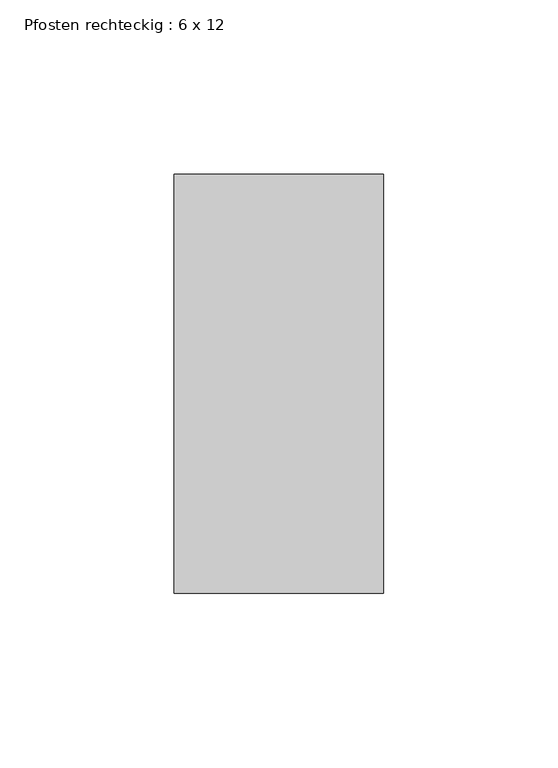
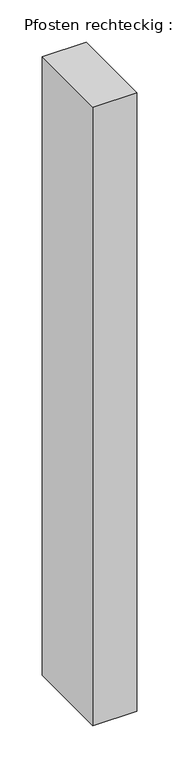
"""IFC4 building model written with IfcOpenShell, lengths in millimetres: member geometry, Pfosten rechteckig : 6 x 12."""

from ifc_helpers import new_model, si_unit, frame, origin, place, context, project, spatial, polyline, outline, extrude, source, transform, mapped, element, save


def pfosten_rechteckig_6_x_12_970216da(model_context):
    return source(origin(), model_context, "Body", "SweptSolid", [
        extrude(outline(polyline([(30.0, 60.0), (30.0, -60.0), (-30.0, -60.0), (-30.0, 60.0), (30.0, 60.0)])), frame((0.0, 0.0, -895.0226945), z_axis=(0.0, 0.0, 1.0), x_axis=(1.0, 0.0, 0.0)), (0.0, 0.0, 1.0), 895.0226945),
    ])


if __name__ == "__main__":
    model = new_model("IFC4")
    model_context = context("Model", 3, world=origin())
    ifc_project = project(units=[si_unit("LENGTHUNIT", "METRE", prefix="MILLI")], contexts=[model_context])
    site = spatial("IfcSite", under=ifc_project)
    building = spatial("IfcBuilding", under=site)
    placement = place(None, origin())
    pfosten_rechteckig_6_x_12_shape = pfosten_rechteckig_6_x_12_970216da(model_context)
    element("IfcMember", 1, ObjectType="Pfosten rechteckig : 6 x 12", at=placement, inside=building, context=model_context, shape_type="MappedRepresentation", body=[
        mapped(pfosten_rechteckig_6_x_12_shape, transform((0.0, 0.0, 0.0), x_axis=(1.0, 0.0, 0.0), y_axis=(0.0, 1.0, 0.0), z_axis=(0.0, 0.0, 1.0))),
    ])
    save(model, "model.ifc")

# Revit data of these elements
# Type "Pfosten rechteckig : 6 x 12"
#   built-in parameter 1007304 = 0.393701 (stored number, unit not read)
#   built-in parameter 1007301 = 0.0984252 (stored number, unit not read)
#   built-in parameter 1007300 = 0.0984252 (stored number, unit not read)
# Element 1 (IfcMember, "Pfosten rechteckig : 6 x 12")
#   Materials on its faces: "Metall - verzinkt"
# Materials
#   "Metall - verzinkt": class "Allgemeines", colour RGB 200 200 200, transparency 0, Cost = 0
